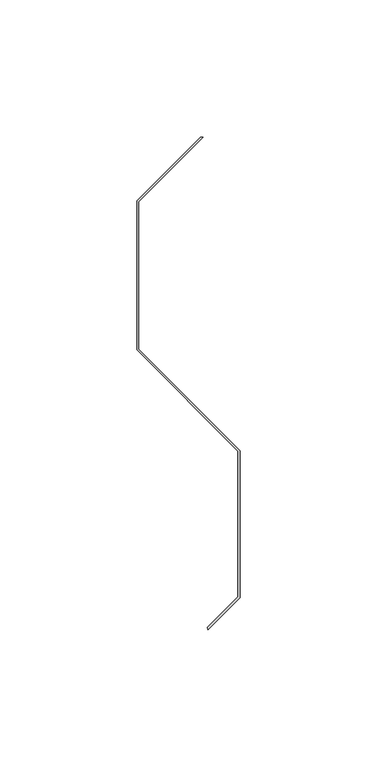
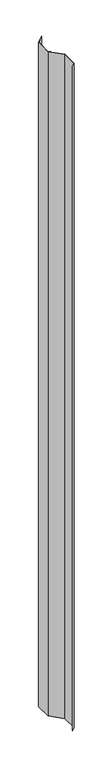
"""IFC4 building model written with IfcOpenShell, lengths in millimetres: proxy geometry, MBCI 7.2-V Panel38 : MBCI 7.2-V Panel-1."""

from ifc_helpers import new_model, si_unit, frame, origin, place, context, project, spatial, polyline, outline, extrude, source, transform, mapped, element, save


def generic_models_c199058d(model_context):
    return source(origin(), model_context, "Body", "SweptSolid", [
        extrude(outline(polyline([(587367.6508364, -533005.919184), (587367.6508364, -533059.500484), (587355.9801137, -533071.1712068), (587355.92509, -533070.3843314), (587367.0555239, -533059.2538975), (587367.0555239, -533006.1657706), (587330.1604364, -532969.2706831), (587330.1604364, -532914.9900192), (587353.3965716, -532891.7538841), (587354.2384706, -532891.7538841), (587330.7557489, -532915.2366057), (587330.7557489, -532969.0240965), (587367.6508364, -533005.919184)])), frame((0.0, 0.0, 51.59375), z_axis=(0.0, 0.0, 1.0), x_axis=(1.0, 0.0, 0.0)), (0.0, 0.0, 1.0), 2386.80625),
    ])


if __name__ == "__main__":
    model = new_model("IFC4")
    model_context = context("Model", 3, world=origin())
    ifc_project = project(units=[si_unit("LENGTHUNIT", "METRE", prefix="MILLI")], contexts=[model_context])
    site = spatial("IfcSite", under=ifc_project)
    building = spatial("IfcBuilding", under=site)
    placement = place(None, origin())
    generic_models_shape = generic_models_c199058d(model_context)
    element("IfcBuildingElementProxy", 1, Name="MBCI 7.2-V Panel38 : MBCI 7.2-V Panel-1", ObjectType="MBCI 7.2-V Panel38 : MBCI 7.2-V Panel-1", at=placement, inside=building, context=model_context, shape_type="MappedRepresentation", body=[
        mapped(generic_models_shape, transform((0.0, 0.0, 0.0), x_axis=(1.0, 0.0, 0.0), y_axis=(0.0, 1.0, 0.0), z_axis=(0.0, 0.0, 1.0))),
    ])
    save(model, "model.ifc")

# Revit data of these elements
# Element 1 (IfcBuildingElementProxy, "MBCI 7.2-V Panel38 : MBCI 7.2-V Panel-1")
#   Materials on its faces: "MTL PANEL"
# Materials
#   "MTL PANEL": class "Generic", colour RGB 239 242 240, transparency 0, Cost = 0
